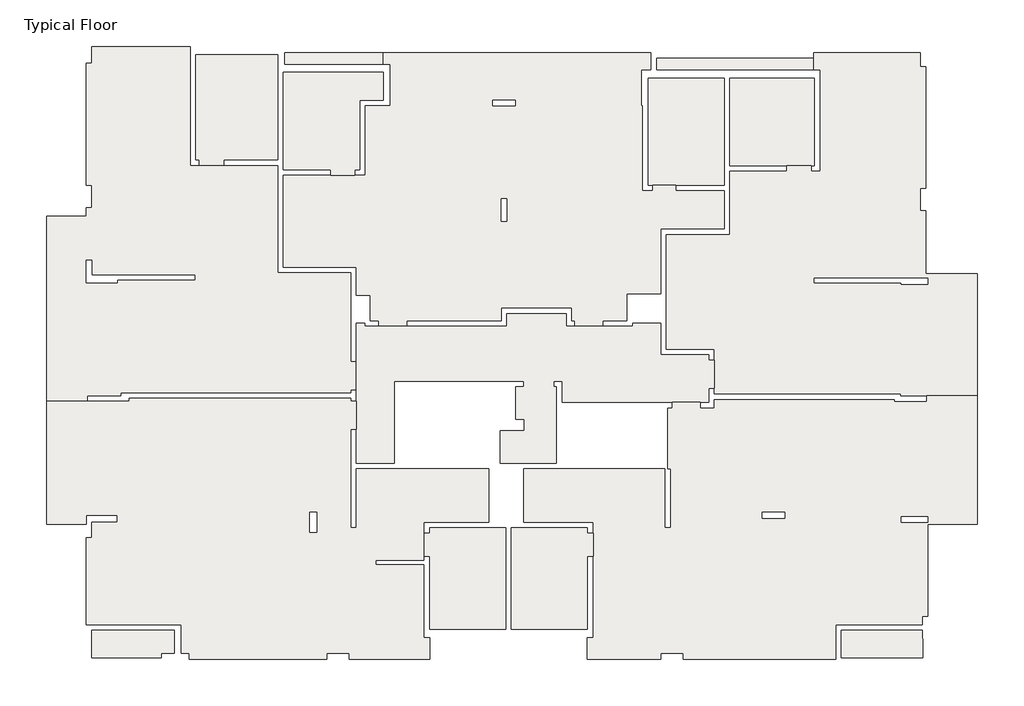
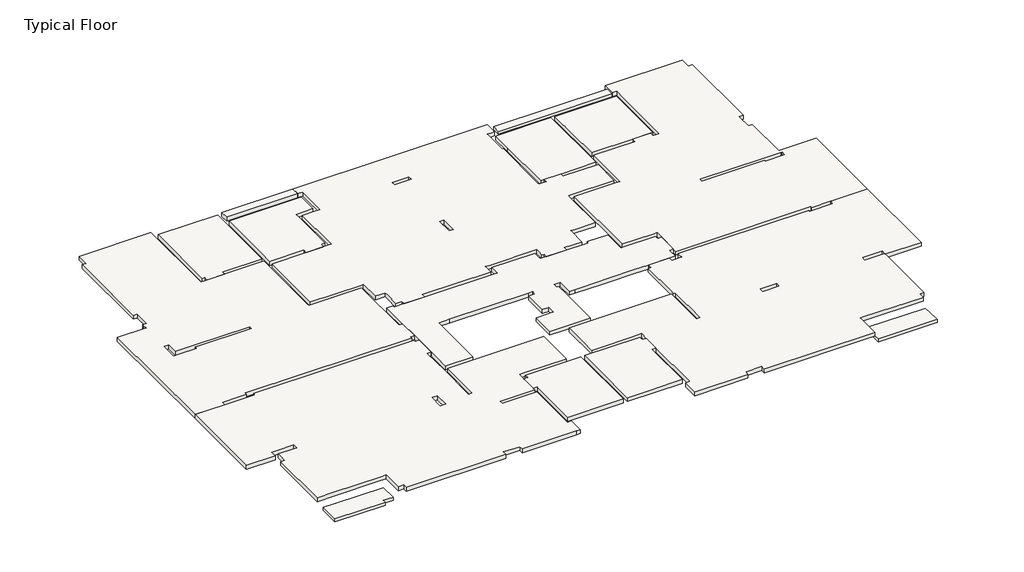
# One storey: 16 slabs.
# Revit data of these elements (continued)
# Element 7 (IfcSlab, "20") (continued)
#   built-in parameter 1001954 = 1
#   SOFiSTiK_AMG_Scheduled = yes
#   SOFiSTiK_AMG_Adjusted = yes
#   Phase Created = New Construction
#   Materials on its faces: "Concrete"
# Element 8 (IfcSlab, "20")
#   Mark = "S5"
#   SOFiSTiK_AMG_Comments = ""
#   Height Offset From Level = 0 cm
#   built-in parameter 1001954 = 1
#   SOFiSTiK_AMG_Scheduled = yes
#   SOFiSTiK_AMG_Adjusted = yes
#   Phase Created = New Construction
#   Materials on its faces: "Concrete"
# Element 9 (IfcSlab, "20")
#   Mark = "S6"
#   SOFiSTiK_AMG_Comments = ""
#   built-in parameter 1001955 = 1.5708 (stored number, unit not read)
#   Height Offset From Level = 0 cm
#   built-in parameter 1001954 = 1
#   SOFiSTiK_AMG_Scheduled = yes
#   SOFiSTiK_AMG_Adjusted = yes
#   Phase Created = New Construction
#   Materials on its faces: "Concrete"
# Element 10 (IfcSlab, "20")
#   Mark = "S7"
#   SOFiSTiK_AMG_Comments = ""
#   built-in parameter 1001955 = 3.14159 (stored number, unit not read)
#   Height Offset From Level = 0 cm
#   built-in parameter 1001954 = 1
#   SOFiSTiK_AMG_Scheduled = yes
#   SOFiSTiK_AMG_Adjusted = yes
#   Phase Created = New Construction
#   Materials on its faces: "Concrete"
# Element 11 (IfcSlab, "20")
#   Mark = "S8"
#   SOFiSTiK_AMG_Comments = ""
#   Height Offset From Level = 0 cm
#   built-in parameter 1001954 = 1
#   SOFiSTiK_AMG_Scheduled = yes
#   SOFiSTiK_AMG_Adjusted = yes
#   Phase Created = New Construction
#   Materials on its faces: "Concrete"
# Element 12 (IfcSlab, "20")
#   Mark = "S9"
#   SOFiSTiK_AMG_Comments = ""
#   built-in parameter 1001955 = 3.14159 (stored number, unit not read)
#   Height Offset From Level = 0 cm
#   built-in parameter 1001954 = 1
#   SOFiSTiK_AMG_Scheduled = yes
#   SOFiSTiK_AMG_Adjusted = yes
#   Phase Created = New Construction
#   Materials on its faces: "Concrete"
# Element 13 (IfcSlab, "20")
#   Mark = "S10"
#   SOFiSTiK_AMG_Comments = ""
#   built-in parameter 1001955 = -1.5708 (stored number, unit not read)
#   Height Offset From Level = 0 cm
#   built-in parameter 1001954 = 1
#   SOFiSTiK_AMG_Scheduled = yes
#   SOFiSTiK_AMG_Adjusted = no
#   Phase Created = New Construction
#   Materials on its faces: "Concrete"
# Element 14 (IfcSlab, "20")
#   Mark = "S11"
#   SOFiSTiK_AMG_Comments = ""
#   Height Offset From Level = 0 cm
#   built-in parameter 1001954 = 1
#   SOFiSTiK_AMG_Scheduled = yes
#   SOFiSTiK_AMG_Adjusted = no
#   Phase Created = New Construction
#   Materials on its faces: "Concrete"
# Element 15 (IfcSlab, "20")
#   Mark = "S12"
#   SOFiSTiK_AMG_Comments = ""
#   Height Offset From Level = 0 cm
#   built-in parameter 1001954 = 1
#   SOFiSTiK_AMG_Scheduled = yes
#   SOFiSTiK_AMG_Adjusted = yes
#   Phase Created = New Construction
#   Materials on its faces: "Concrete"
# Element 16 (IfcSlab, "20")
#   Mark = "S13"
#   SOFiSTiK_AMG_Comments = ""
#   Height Offset From Level = 0 cm
#   built-in parameter 1001954 = 1
#   SOFiSTiK_AMG_Scheduled = yes
#   SOFiSTiK_AMG_Adjusted = yes
#   Phase Created = New Construction
#   Materials on its faces: "Concrete"
# Materials
#   "Concrete": class "Concrete", colour RGB 192 192 192, transparency 0, Keynote = "01000", Description = "Cast-in-place concrete", Cost = 0
